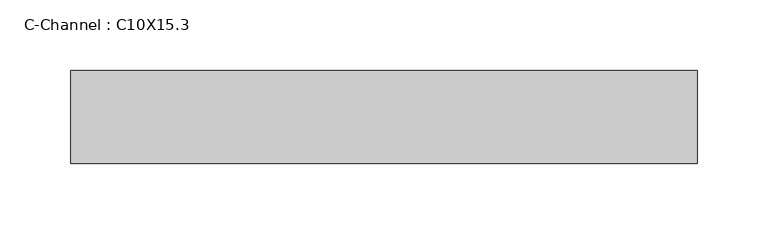
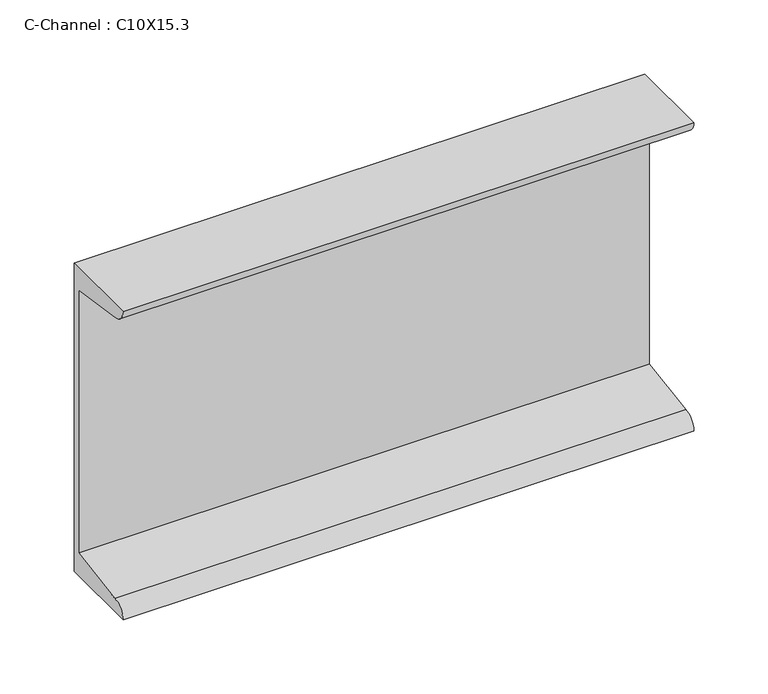
"""IFC4 building model written with IfcOpenShell, lengths in millimetres: beam geometry, C-Channel : C10X15.3."""

from ifc_helpers import new_model, si_unit, point, frame, frame_2d, origin, place, context, project, spatial, polyline, circle_curve, trimmed, segment, composite_curve, outline, extrude, source, transform, mapped, element, save


def c_channel_c10x15_3_3b942c7d(model_context):
    return source(origin(), model_context, "Body", "SweptSolid", [
        extrude(outline(composite_curve([segment(polyline([(16.1036, 127.0), (16.1036, -127.0), (-49.9364, -127.0)]), True, "CONTINUOUS"), segment(trimmed(circle_curve(frame_2d((-38.862, -127.0)), 11.0744), [point((-49.9364, -127.0))], [point((-38.862, -115.9256))], False, "CARTESIAN"), True, "CONTINUOUS"), segment(polyline([(-38.862, -115.9256), (10.0076, -108.1854158), (10.0076, 108.1854158), (-38.862, 115.9256)]), True, "CONTINUOUS"), segment(trimmed(circle_curve(frame_2d((-38.862, 127.0)), 11.0744), [point((-38.862, 115.9256))], [point((-49.9364, 127.0))], False, "CARTESIAN"), True, "CONTINUOUS"), segment(polyline([(-49.9364, 127.0), (16.1036, 127.0)]), True, "CONTINUOUS")], self_intersect=False)), frame((-292.1, 0.0, 0.0), z_axis=(1.0, 0.0, 0.0), x_axis=(0.0, 1.0, 0.0)), (0.0, 0.0, 1.0), 444.5),
    ])


if __name__ == "__main__":
    model = new_model("IFC4")
    model_context = context("Model", 3, world=origin())
    ifc_project = project(units=[si_unit("LENGTHUNIT", "METRE", prefix="MILLI")], contexts=[model_context])
    site = spatial("IfcSite", under=ifc_project)
    building = spatial("IfcBuilding", under=site)
    placement = place(None, origin())
    c_channel_c10x15_3_shape = c_channel_c10x15_3_3b942c7d(model_context)
    element("IfcBeam", 1, ObjectType="C-Channel : C10X15.3", at=placement, inside=building, context=model_context, shape_type="MappedRepresentation", body=[
        mapped(c_channel_c10x15_3_shape, transform((0.0, 0.0, 0.0), x_axis=(1.0, 0.0, 0.0), y_axis=(0.0, 1.0, 0.0), z_axis=(0.0, 0.0, 1.0))),
    ])
    save(model, "model.ifc")

# Revit data of these elements
# Type "C-Channel : C10X15.3"
#   Assembly Code = "B10"
#   W = 15.3
#   Length [instance default] = 5' - 0"
#   bf = 0' - 2.6"
#   d = 0' - 10"
#   tf = 0' - 0.436"
#   tw = 0' - 0.24"
#   x = 0' - 0.634"
#   A = 0.0311111 SF
#   Structural Material [instance default] = Steel ASTM A36
# Element 1 (IfcBeam, "C-Channel : C10X15.3")
#   Structural Material = Steel ASTM A992
#   Materials on its faces: "Steel ASTM A992"
# Materials
#   "Steel ASTM A36": class "Metal", colour RGB 199 199 199, transparency 0, Description = "Structural steel, ASTM A36 Grade B, mill finish", Cost = 0
#   "Steel ASTM A992": class "Metal", colour RGB 199 199 199, transparency 0, Description = "Structural steel 50ksi", Cost = 0
